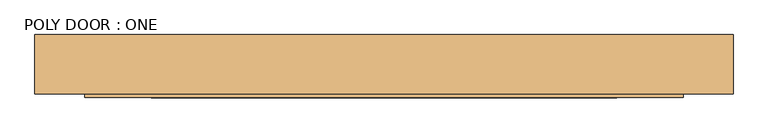
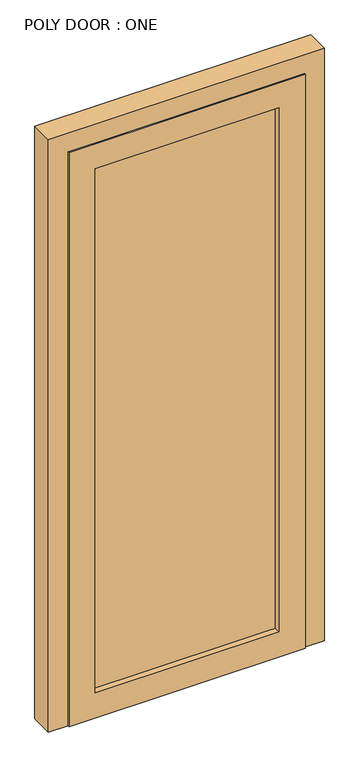
"""IFC4 building model written with IfcOpenShell, lengths in millimetres: door geometry, POLY DOOR : ONE."""

from ifc_helpers import new_model, si_unit, frame, origin, place, context, project, spatial, polyline, outline, extrude, source, transform, mapped, element, save


def poly_door_one_b4ab5f43(model_context):
    return source(origin(), model_context, "Body", "SweptSolid", [
        extrude(outline(polyline([(355.6, -25.4), (-355.6, -25.4), (-355.6, -12.7), (355.6, -12.7), (355.6, -25.4)])), frame((0.0, 0.0, 101.6), z_axis=(0.0, 0.0, 1.0), x_axis=(1.0, 0.0, 0.0)), (0.0, 0.0, 1.0), 2139.95),
        extrude(outline(polyline([(2343.15, 457.2), (2343.15, -457.2), (0.0, -457.2), (0.0, 457.2), (2343.15, 457.2)]), holes=[polyline([(2241.55, 355.6), (101.6, 355.6), (101.6, -355.6), (2241.55, -355.6), (2241.55, 355.6)])]), frame((0.0, -50.8, 0.0), z_axis=(0.0, 1.0, 0.0), x_axis=(0.0, 0.0, 1.0)), (0.0, 0.0, 1.0), 50.8),
        extrude(outline(polyline([(2419.35, -533.4), (0.0, -533.4), (0.0, -457.2), (2343.15, -457.2), (2343.15, 457.2), (0.0, 457.2), (0.0, 533.4), (2419.35, 533.4), (2419.35, -533.4)])), frame((0.0, -45.39996, 0.0), z_axis=(0.0, 1.0, 0.0), x_axis=(0.0, 0.0, 1.0)), (0.0, 0.0, 1.0), 90.79992),
    ])


if __name__ == "__main__":
    model = new_model("IFC4")
    model_context = context("Model", 3, world=origin())
    ifc_project = project(units=[si_unit("LENGTHUNIT", "METRE", prefix="MILLI")], contexts=[model_context])
    site = spatial("IfcSite", under=ifc_project)
    building = spatial("IfcBuilding", under=site)
    placement = place(None, origin())
    poly_door_one_shape = poly_door_one_b4ab5f43(model_context)
    element("IfcDoor", 1, ObjectType="POLY DOOR : ONE", at=placement, inside=building, context=model_context, shape_type="MappedRepresentation", body=[
        mapped(poly_door_one_shape, transform((0.0, 0.0, 0.0), x_axis=(1.0, 0.0, 0.0), y_axis=(0.0, 1.0, 0.0), z_axis=(0.0, 0.0, 1.0))),
    ])
    save(model, "model.ifc")

# Revit data of these elements
# Type "POLY DOOR : ONE"
#   Type Mark = "53"
#   Assembly Code = "C1020"
#   Analytic Construction = "<None>"
#   Thickness = 0' - 2"
#   Glass Inset = 0' - 4"
#   Height = 7' - 8 1/4"
#   Trim Projection Ext = 0' - 1"
#   Trim Projection Int = 0' - 1"
#   Trim Width = 0' - 3"
#   Width = 3' - 0"
#   WINDOW = yes
#   Glass Material = ALUM. STOREFRONT W/ INSULATED GLAZING
#   Door Material = Aluminum
#   Frame Material = Aluminum
#   Function = (empty or 0)
#   Wall Closure = (empty or 0)
# Element 1 (IfcDoor, "POLY DOOR : ONE")
#   Materials on its faces: "Aluminum", "ALUM. STOREFRONT W/ INSULATED GLAZING"
# Materials
#   "ALUM. STOREFRONT W/ INSULATED GLAZING": class "Glass", colour RGB 196 205 210, transparency 0.85, Description = "Soda Lime Glass", Cost = 0
#   "Aluminum": class "Metal", colour RGB 244 244 244, transparency 0, Description = "Aluminum 6061", Cost = 0
